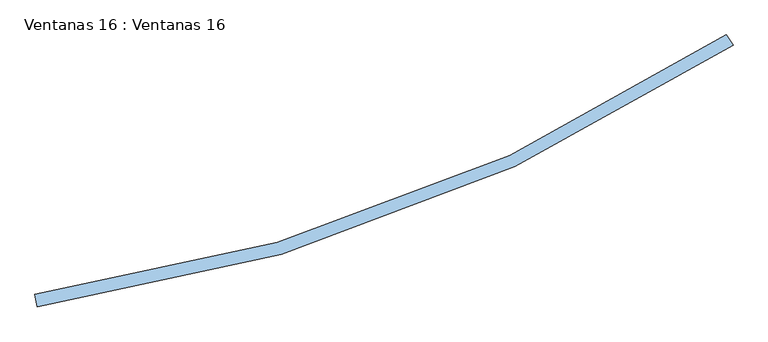
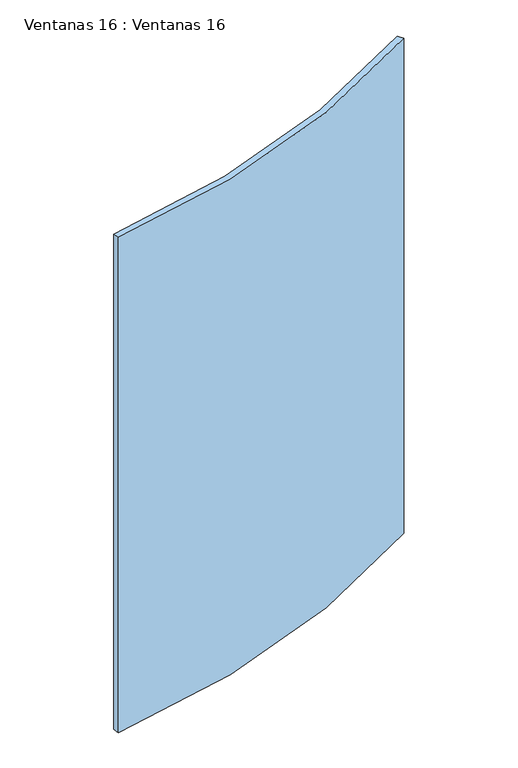
"""IFC4 building model written with IfcOpenShell, lengths in millimetres: window geometry, Ventanas 16 : Ventanas 16."""

from ifc_helpers import new_model, si_unit, point, frame, frame_2d, origin, place, context, project, spatial, polyline, circle_curve, trimmed, segment, composite_curve, outline, extrude, source, transform, mapped, element, save


def ventanas_16_ventanas_16_af499c45(model_context):
    return source(origin(), model_context, "Body", "SweptSolid", [
        extrude(outline(composite_curve([segment(polyline([(-3726.1248587, 4848.0713427), (-3715.275057, 4831.2700986)]), True, "CONTINUOUS"), segment(trimmed(circle_curve(frame_2d((-5196.7699578, 7081.6878294)), 2694.2915774), [point((-3715.275057, 4831.2700986))], [point((-4828.2669966, 4412.7156168))], False, "CARTESIAN"), True, "CONTINUOUS"), segment(polyline([(-4828.2669966, 4412.7156168), (-4831.7399601, 4432.4117719)]), True, "CONTINUOUS"), segment(trimmed(circle_curve(frame_2d((-5196.9036809, 7081.9582205)), 2674.5917308), [point((-4831.7399601, 4432.4117719))], [point((-3726.1248587, 4848.0713427))], True, "CARTESIAN"), True, "CONTINUOUS")], self_intersect=False)), frame((0.0, 0.0, 8172.7171527), z_axis=(0.0, 0.0, 1.0), x_axis=(1.0, 0.0, 0.0)), (0.0, 0.0, 1.0), 1598.0350335),
    ])


if __name__ == "__main__":
    model = new_model("IFC4")
    model_context = context("Model", 3, world=origin())
    ifc_project = project(units=[si_unit("LENGTHUNIT", "METRE", prefix="MILLI")], contexts=[model_context])
    site = spatial("IfcSite", under=ifc_project)
    building = spatial("IfcBuilding", under=site)
    placement = place(None, origin())
    ventanas_16_ventanas_16_shape = ventanas_16_ventanas_16_af499c45(model_context)
    element("IfcWindow", 1, ObjectType="Ventanas 16 : Ventanas 16", at=placement, inside=building, context=model_context, shape_type="MappedRepresentation", body=[
        mapped(ventanas_16_ventanas_16_shape, transform((0.0, 0.0, 0.0), x_axis=(1.0, 0.0, 0.0), y_axis=(0.0, 1.0, 0.0), z_axis=(0.0, 0.0, 1.0))),
    ])
    save(model, "model.ifc")

# Revit data of these elements
# Type "Ventanas 16 : Ventanas 16"
#   Type Mark = "42"
# Element 1 (IfcWindow, "Ventanas 16 : Ventanas 16")
#   Materials on its faces: "VIDRIO"
# Materials
#   "VIDRIO": class "Genérico", colour RGB 120 120 120, transparency 0, Cost = 0
